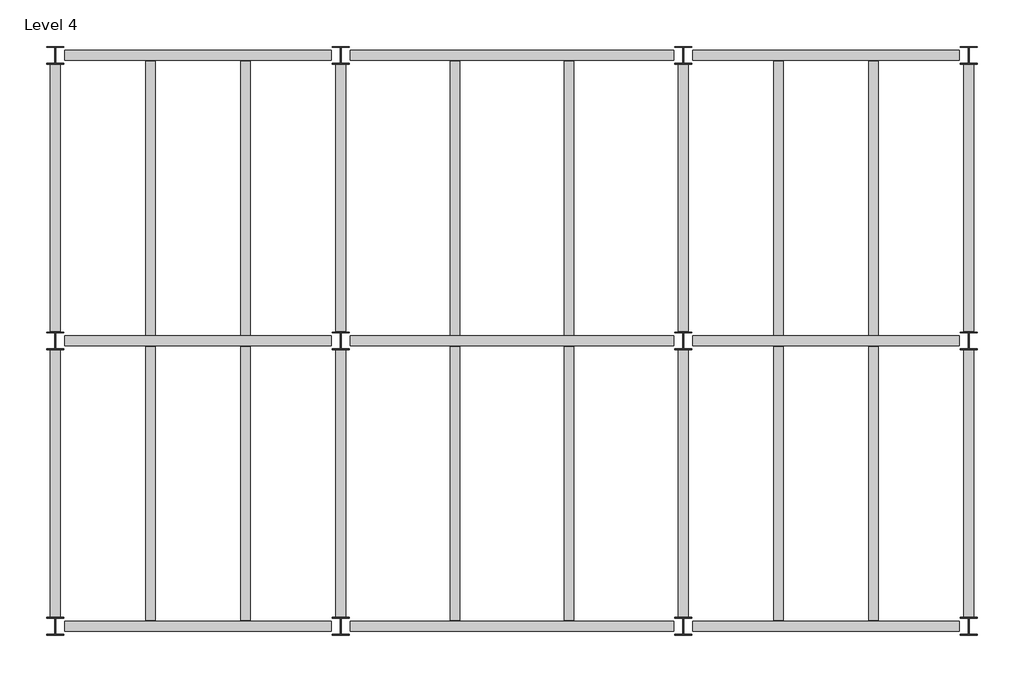
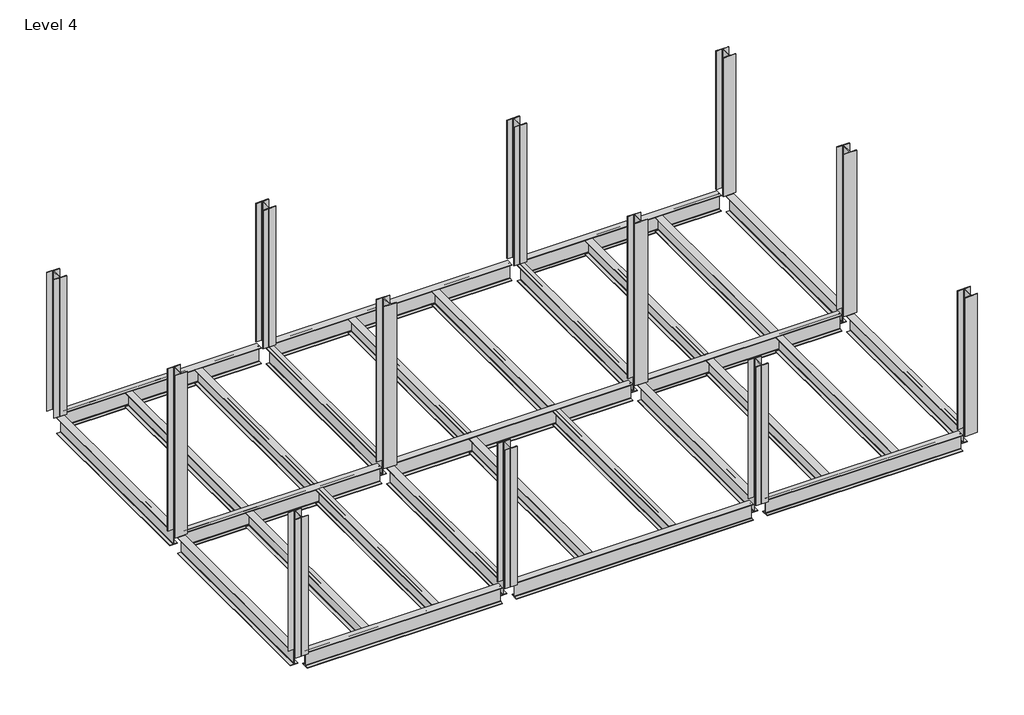
# One storey: 29 beams, 12 columns.
"""IFC4 building model written with IfcOpenShell, lengths in millimetres."""

import ifcopenshell
import ifcopenshell.guid

model = None  # the IFC model being written
_history = None  # IfcOwnerHistory: only IFC2X3 demands one
_inside = {}  # id of a spatial element -> (the spatial element, [elements in it])
_under = {}  # id of a project, library or spatial element -> (it, [spatial elements below it])
_declared = {}  # id of a project -> (the project, [libraries it declares])
_typed = {}  # id of a type object -> (the type object, [elements of that type])
_made_of = {}  # id of a material, layer set ... -> (it, [elements and type objects made of it])


def new_model(schema):
    """Start an empty IFC model of exactly this schema.

    Asked for "IFC4X3", IfcOpenShell would pick the latest addendum, in which some entities
    have other attributes; the version numbers below select the first issue.
    IFC2X3 requires an IfcOwnerHistory on every rooted entity: one is made here for all.
    """
    global model, _history
    if schema == "IFC4X3":
        model = ifcopenshell.file(schema_version=(4, 3, 0, 0))
    else:
        model = ifcopenshell.file(schema=schema)
    _inside.clear()
    _under.clear()
    _declared.clear()
    _typed.clear()
    _made_of.clear()
    _history = None
    if model.schema == "IFC2X3":
        org = make("IfcOrganization", Name="unknown")
        user = make(
            "IfcPersonAndOrganization",
            ThePerson=make("IfcPerson", FamilyName="unknown"),
            TheOrganization=org,
        )
        app = make(
            "IfcApplication",
            ApplicationDeveloper=org,
            Version="unknown",
            ApplicationFullName="unknown",
            ApplicationIdentifier="unknown",
        )
        _history = make(
            "IfcOwnerHistory",
            OwningUser=user,
            OwningApplication=app,
            ChangeAction="ADDED",
            CreationDate=0,
        )
    return model


def make(cls, **values):
    """One entity of the class cls with the attributes given. An attribute that is None is left unset."""
    return model.create_entity(
        cls, **{name: value for name, value in values.items() if value is not None}
    )


def rooted(cls, **values):
    """An entity with a GlobalId (a new one), such as an element, a storey or a relation."""
    return make(cls, GlobalId=ifcopenshell.guid.new(), OwnerHistory=_history, **values)


def si_unit(unit_type, name, prefix=None):
    """IfcSIUnit, for example si_unit("LENGTHUNIT", "METRE", prefix="MILLI")."""
    return make("IfcSIUnit", UnitType=unit_type, Prefix=prefix, Name=name)


def assignment(units):
    """IfcUnitAssignment: the units of a project."""
    return None if units is None else make("IfcUnitAssignment", Units=units)


def point(xyz):
    """IfcCartesianPoint."""
    return None if xyz is None else make("IfcCartesianPoint", Coordinates=xyz)


def direction(xyz):
    """IfcDirection."""
    return None if xyz is None else make("IfcDirection", DirectionRatios=xyz)


def frame(location, z_axis=None, x_axis=None):
    """IfcAxis2Placement3D, a coordinate frame: its origin and axes. An axis left out is left unset."""
    return make(
        "IfcAxis2Placement3D",
        Location=point(location),
        Axis=direction(z_axis),
        RefDirection=direction(x_axis),
    )


def frame_2d(location, x_axis=None):
    """IfcAxis2Placement2D, a coordinate frame in the plane: its origin and x axis."""
    return make(
        "IfcAxis2Placement2D", Location=point(location), RefDirection=direction(x_axis)
    )


def origin():
    """The frame at (0, 0, 0) with its axes left unset."""
    return frame((0.0, 0.0, 0.0))


def place(relative_to, where):
    """IfcLocalPlacement: puts the frame where relative to a parent placement (None: the world)."""
    return make(
        "IfcLocalPlacement", PlacementRelTo=relative_to, RelativePlacement=where
    )


def context(
    kind, dimensions, precision=None, world=None, true_north=None, identifier=None
):
    """IfcGeometricRepresentationContext, for example the 3D "Model" context."""
    return make(
        "IfcGeometricRepresentationContext",
        ContextIdentifier=identifier,
        ContextType=kind,
        CoordinateSpaceDimension=dimensions,
        Precision=precision,
        WorldCoordinateSystem=world,
        TrueNorth=true_north,
    )


def project(units=None, contexts=None):
    """IfcProject with its units and contexts."""
    return rooted(
        "IfcProject",
        Name="project",
        RepresentationContexts=contexts,
        UnitsInContext=assignment(units),
    )


def spatial(cls, under=None, at=None, **own):
    """A site, building, storey or space (cls), placed at a placement, below another one or the project."""
    s = rooted(cls, ObjectPlacement=at, **own)
    if under is not None:
        _under.setdefault(under.id(), (under, []))[1].append(s)
    return s


def polyline(points):
    """IfcPolyline through the points."""
    return make("IfcPolyline", Points=[point(p) for p in points])


def circle_curve(where, radius):
    """IfcCircle in the frame where."""
    return make("IfcCircle", Position=where, Radius=radius)


def trimmed(basis, trim1, trim2, sense, master):
    """IfcTrimmedCurve: the piece of a basis curve between two trims."""
    return make(
        "IfcTrimmedCurve",
        BasisCurve=basis,
        Trim1=trim1,
        Trim2=trim2,
        SenseAgreement=sense,
        MasterRepresentation=master,
    )


def segment(curve, same_sense, transition):
    """IfcCompositeCurveSegment."""
    return make(
        "IfcCompositeCurveSegment",
        Transition=transition,
        SameSense=same_sense,
        ParentCurve=curve,
    )


def composite_curve(segments, self_intersect=None):
    """IfcCompositeCurve: segments joined end to end."""
    return make("IfcCompositeCurve", Segments=segments, SelfIntersect=self_intersect)


def outline(outer, holes=None, kind="AREA"):
    """IfcArbitraryClosedProfileDef: a profile drawn as a closed curve; with holes, ...WithVoids."""
    if holes is None:
        return make("IfcArbitraryClosedProfileDef", ProfileType=kind, OuterCurve=outer)
    return make(
        "IfcArbitraryProfileDefWithVoids",
        ProfileType=kind,
        OuterCurve=outer,
        InnerCurves=holes,
    )


def extrude(swept, where, along, depth):
    """IfcExtrudedAreaSolid: the profile swept, set in the frame where, extruded along a direction by depth."""
    return make(
        "IfcExtrudedAreaSolid",
        SweptArea=swept,
        Position=where,
        ExtrudedDirection=direction(along),
        Depth=depth,
    )


def shape(context_of_items, identifier, shape_type, items):
    """IfcShapeRepresentation: the items that make up one representation, for example the "Body"."""
    return make(
        "IfcShapeRepresentation",
        ContextOfItems=context_of_items,
        RepresentationIdentifier=identifier,
        RepresentationType=shape_type,
        Items=items,
    )


def source(mapping_origin, context_of_items, identifier, shape_type, items):
    """IfcRepresentationMap: a shape defined once, which mapped items show again and again."""
    return make(
        "IfcRepresentationMap",
        MappingOrigin=mapping_origin,
        MappedRepresentation=shape(context_of_items, identifier, shape_type, items),
    )


def transform(
    local_origin,
    x_axis=None,
    y_axis=None,
    z_axis=None,
    scale=None,
    scale2=None,
    scale3=None,
    uniform=True,
):
    """IfcCartesianTransformationOperator3D, or its non-uniform kind. x_axis, y_axis, z_axis: its Axis1, 2, 3."""
    if uniform:
        return make(
            "IfcCartesianTransformationOperator3D",
            Axis1=direction(x_axis),
            Axis2=direction(y_axis),
            LocalOrigin=point(local_origin),
            Scale=scale,
            Axis3=direction(z_axis),
        )
    return make(
        "IfcCartesianTransformationOperator3DnonUniform",
        Axis1=direction(x_axis),
        Axis2=direction(y_axis),
        LocalOrigin=point(local_origin),
        Scale=scale,
        Axis3=direction(z_axis),
        Scale2=scale2,
        Scale3=scale3,
    )


def mapped(mapping_source, mapping_target):
    """IfcMappedItem: shows the shape of a source again, moved by a transform."""
    return make(
        "IfcMappedItem", MappingSource=mapping_source, MappingTarget=mapping_target
    )


def made_of(thing, what):
    """Note that an element or type object is made of a material, layer set ...; save() writes the relation."""
    if what is not None:
        _made_of.setdefault(what.id(), (what, []))[1].append(thing)
    return thing


def element(
    cls,
    number,
    at=None,
    inside=None,
    cuts=None,
    type_object=None,
    material=None,
    context=None,
    identifier="Body",
    shape_type=None,
    held_by="IfcProductDefinitionShape",
    body=None,
    shapes=None,
    **own,
):
    """One element of the class cls, such as IfcWall. Its Tag is "e" and its number.

    at: its placement. inside: the storey or other place that contains it. cuts: it is an
    opening in that element (IfcRelVoidsElement). A single representation is given by context,
    identifier, shape_type and body (its items); several are given by shapes. held_by: the class
    of the entity that holds the representations. save() writes the other relations.
    """
    e = rooted(cls, Tag="e%d" % number, ObjectPlacement=at, **own)
    if body is not None:
        shapes = [shape(context, identifier, shape_type, body)]
    if shapes is not None:
        e.Representation = make(held_by, Representations=shapes)
    if inside is not None:
        _inside.setdefault(inside.id(), (inside, []))[1].append(e)
    if cuts is not None:
        rooted(
            "IfcRelVoidsElement", RelatingBuildingElement=cuts, RelatedOpeningElement=e
        )
    if type_object is not None:
        _typed.setdefault(type_object.id(), (type_object, []))[1].append(e)
    return made_of(e, material)


def aggregate(whole, parts):
    """IfcRelAggregates: a whole, such as a stair, and the parts it consists of."""
    return rooted("IfcRelAggregates", RelatingObject=whole, RelatedObjects=parts)


def save(model, path):
    """Write the relations noted so far, then the file.

    IfcRelAggregates (storeys below a building ...), IfcRelContainedInSpatialStructure (elements
    in a storey), IfcRelDefinesByType, IfcRelAssociatesMaterial and IfcRelDeclares: one each for
    every whole, place, type object, material and project.
    """
    for whole, parts in _under.values():
        aggregate(whole, parts)
    for where, things in _inside.values():
        rooted(
            "IfcRelContainedInSpatialStructure",
            RelatedElements=things,
            RelatingStructure=where,
        )
    for kind, things in _typed.values():
        rooted("IfcRelDefinesByType", RelatedObjects=things, RelatingType=kind)
    for what, things in _made_of.values():
        rooted("IfcRelAssociatesMaterial", RelatedObjects=things, RelatingMaterial=what)
    for by, libraries in _declared.values():
        rooted("IfcRelDeclares", RelatingContext=by, RelatedDefinitions=libraries)
    model.write(path)


def ub_universal_beams_ub356x171x51_26e98692(model_context):
    return source(origin(), model_context, "Body", "SweptSolid", [
        extrude(outline(composite_curve([segment(polyline([(85.75, -166.0), (85.75, -177.5), (-85.75, -177.5), (-85.75, -166.0), (-13.9, -166.0)]), True, "CONTINUOUS"), segment(trimmed(circle_curve(frame_2d((-13.9, -155.8)), 10.2), [point((-13.9, -166.0))], [point((-3.7, -155.8))], True, "CARTESIAN"), True, "CONTINUOUS"), segment(polyline([(-3.7, -155.8), (-3.7, 155.8)]), True, "CONTINUOUS"), segment(trimmed(circle_curve(frame_2d((-13.9, 155.8)), 10.2), [point((-3.7, 155.8))], [point((-13.9, 166.0))], True, "CARTESIAN"), True, "CONTINUOUS"), segment(polyline([(-13.9, 166.0), (-85.75, 166.0), (-85.75, 177.5), (85.75, 177.5), (85.75, 166.0), (13.9, 166.0)]), True, "CONTINUOUS"), segment(trimmed(circle_curve(frame_2d((13.9, 155.8)), 10.2), [point((13.9, 166.0))], [point((3.7, 155.8))], True, "CARTESIAN"), True, "CONTINUOUS"), segment(polyline([(3.7, 155.8), (3.7, -155.8)]), True, "CONTINUOUS"), segment(trimmed(circle_curve(frame_2d((13.9, -155.8)), 10.2), [point((3.7, -155.8))], [point((13.9, -166.0))], True, "CARTESIAN"), True, "CONTINUOUS"), segment(polyline([(13.9, -166.0), (85.75, -166.0)]), True, "CONTINUOUS")], self_intersect=False)), frame((-2398.3, 0.0, 0.0), z_axis=(1.0, 0.0, 0.0), x_axis=(0.0, 1.0, 0.0)), (0.0, 0.0, 1.0), 4796.6),
    ])


def ub_universal_beams_ub406x178x60_425a89a6(model_context):
    return source(origin(), model_context, "Body", "SweptSolid", [
        extrude(outline(composite_curve([segment(polyline([(88.95, -190.4), (88.95, -203.2), (-88.95, -203.2), (-88.95, -190.4), (-14.15, -190.4)]), True, "CONTINUOUS"), segment(trimmed(circle_curve(frame_2d((-14.15, -180.2)), 10.2), [point((-14.15, -190.4))], [point((-3.95, -180.2))], True, "CARTESIAN"), True, "CONTINUOUS"), segment(polyline([(-3.95, -180.2), (-3.95, 180.2)]), True, "CONTINUOUS"), segment(trimmed(circle_curve(frame_2d((-14.15, 180.2)), 10.2), [point((-3.95, 180.2))], [point((-14.15, 190.4))], True, "CARTESIAN"), True, "CONTINUOUS"), segment(polyline([(-14.15, 190.4), (-88.95, 190.4), (-88.95, 203.2), (88.95, 203.2), (88.95, 190.4), (14.15, 190.4)]), True, "CONTINUOUS"), segment(trimmed(circle_curve(frame_2d((14.15, 180.2)), 10.2), [point((14.15, 190.4))], [point((3.95, 180.2))], True, "CARTESIAN"), True, "CONTINUOUS"), segment(polyline([(3.95, 180.2), (3.95, -180.2)]), True, "CONTINUOUS"), segment(trimmed(circle_curve(frame_2d((14.15, -180.2)), 10.2), [point((3.95, -180.2))], [point((14.15, -190.4))], True, "CARTESIAN"), True, "CONTINUOUS"), segment(polyline([(14.15, -190.4), (88.95, -190.4)]), True, "CONTINUOUS")], self_intersect=False)), frame((-2334.6, 0.0, 0.0), z_axis=(1.0, 0.0, 0.0), x_axis=(0.0, 1.0, 0.0)), (0.0, 0.0, 1.0), 4669.2),
    ])


def ub_universal_beams_ub406x178x60_ab0c7e2f(model_context):
    return source(origin(), model_context, "Body", "SweptSolid", [
        extrude(outline(composite_curve([segment(polyline([(88.95, -190.4), (88.95, -203.2), (-88.95, -203.2), (-88.95, -190.4), (-14.15, -190.4)]), True, "CONTINUOUS"), segment(trimmed(circle_curve(frame_2d((-14.15, -180.2)), 10.2), [point((-14.15, -190.4))], [point((-3.95, -180.2))], True, "CARTESIAN"), True, "CONTINUOUS"), segment(polyline([(-3.95, -180.2), (-3.95, 180.2)]), True, "CONTINUOUS"), segment(trimmed(circle_curve(frame_2d((-14.15, 180.2)), 10.2), [point((-3.95, 180.2))], [point((-14.15, 190.4))], True, "CARTESIAN"), True, "CONTINUOUS"), segment(polyline([(-14.15, 190.4), (-88.95, 190.4), (-88.95, 203.2), (88.95, 203.2), (88.95, 190.4), (14.15, 190.4)]), True, "CONTINUOUS"), segment(trimmed(circle_curve(frame_2d((14.15, 180.2)), 10.2), [point((14.15, 190.4))], [point((3.95, 180.2))], True, "CARTESIAN"), True, "CONTINUOUS"), segment(polyline([(3.95, 180.2), (3.95, -180.2)]), True, "CONTINUOUS"), segment(trimmed(circle_curve(frame_2d((14.15, -180.2)), 10.2), [point((3.95, -180.2))], [point((14.15, -190.4))], True, "CARTESIAN"), True, "CONTINUOUS"), segment(polyline([(14.15, -190.4), (88.95, -190.4)]), True, "CONTINUOUS")], self_intersect=False)), frame((-2834.6, 0.0, 0.0), z_axis=(1.0, 0.0, 0.0), x_axis=(0.0, 1.0, 0.0)), (0.0, 0.0, 1.0), 5669.2),
    ])


def ub_universal_beams_ub406x178x60_873acc54(model_context):
    return source(origin(), model_context, "Body", "SweptSolid", [
        extrude(outline(composite_curve([segment(polyline([(88.95, -190.4), (88.95, -203.2), (-88.95, -203.2), (-88.95, -190.4), (-14.15, -190.4)]), True, "CONTINUOUS"), segment(trimmed(circle_curve(frame_2d((-14.15, -180.2)), 10.2), [point((-14.15, -190.4))], [point((-3.95, -180.2))], True, "CARTESIAN"), True, "CONTINUOUS"), segment(polyline([(-3.95, -180.2), (-3.95, 180.2)]), True, "CONTINUOUS"), segment(trimmed(circle_curve(frame_2d((-14.15, 180.2)), 10.2), [point((-3.95, 180.2))], [point((-14.15, 190.4))], True, "CARTESIAN"), True, "CONTINUOUS"), segment(polyline([(-14.15, 190.4), (-88.95, 190.4), (-88.95, 203.2), (88.95, 203.2), (88.95, 190.4), (14.15, 190.4)]), True, "CONTINUOUS"), segment(trimmed(circle_curve(frame_2d((14.15, 180.2)), 10.2), [point((14.15, 190.4))], [point((3.95, 180.2))], True, "CARTESIAN"), True, "CONTINUOUS"), segment(polyline([(3.95, 180.2), (3.95, -180.2)]), True, "CONTINUOUS"), segment(trimmed(circle_curve(frame_2d((14.15, -180.2)), 10.2), [point((3.95, -180.2))], [point((14.15, -190.4))], True, "CARTESIAN"), True, "CONTINUOUS"), segment(polyline([(14.15, -190.4), (88.95, -190.4)]), True, "CONTINUOUS")], self_intersect=False)), frame((-2333.3, 0.0, 0.0), z_axis=(1.0, 0.0, 0.0), x_axis=(0.0, 1.0, 0.0)), (0.0, 0.0, 1.0), 4666.6),
    ])


model = new_model("IFC4")

# Units and contexts
model_context = context("Model", 3, world=origin())
ifc_project = project(units=[si_unit("LENGTHUNIT", "METRE", prefix="MILLI")], contexts=[model_context])

# Site, building, storey
site = spatial("IfcSite", under=ifc_project)
building = spatial("IfcBuilding", under=site)
storey = spatial("IfcBuildingStorey", under=building, Name="Level 4", Elevation=9000.0)

# Beams
placement = place(None, origin())
ub_universal_beams_ub356x171x51_shape = ub_universal_beams_ub356x171x51_26e98692(model_context)
element("IfcBeam", 1, ObjectType="UB-Universal Beams : UB356x171x51", at=placement, inside=storey, context=model_context, shape_type="MappedRepresentation", body=[
    mapped(ub_universal_beams_ub356x171x51_shape, transform((1666.6666667, 2500.0, 8822.5), x_axis=(0.0, 1.0, 0.0), y_axis=(-1.0, 0.0, 0.0), z_axis=(0.0, 0.0, 1.0))),
])
element("IfcBeam", 2, ObjectType="UB-Universal Beams : UB356x171x51", at=placement, inside=storey, context=model_context, shape_type="MappedRepresentation", body=[
    mapped(ub_universal_beams_ub356x171x51_shape, transform((3333.3333333, 2500.0, 8822.5), x_axis=(0.0, 1.0, 0.0), y_axis=(-1.0, 0.0, 0.0), z_axis=(0.0, 0.0, 1.0))),
])
element("IfcBeam", 3, ObjectType="UB-Universal Beams : UB356x171x51", at=placement, inside=storey, context=model_context, shape_type="MappedRepresentation", body=[
    mapped(ub_universal_beams_ub356x171x51_shape, transform((7000.0, 2500.0, 8822.5), x_axis=(0.0, 1.0, 0.0), y_axis=(-1.0, 0.0, 0.0), z_axis=(0.0, 0.0, 1.0))),
])
element("IfcBeam", 4, ObjectType="UB-Universal Beams : UB356x171x51", at=placement, inside=storey, context=model_context, shape_type="MappedRepresentation", body=[
    mapped(ub_universal_beams_ub356x171x51_shape, transform((9000.0, 2500.0, 8822.5), x_axis=(0.0, 1.0, 0.0), y_axis=(-1.0, 0.0, 0.0), z_axis=(0.0, 0.0, 1.0))),
])
element("IfcBeam", 5, ObjectType="UB-Universal Beams : UB356x171x51", at=placement, inside=storey, context=model_context, shape_type="MappedRepresentation", body=[
    mapped(ub_universal_beams_ub356x171x51_shape, transform((12666.6666667, 2500.0, 8822.5), x_axis=(0.0, 1.0, 0.0), y_axis=(-1.0, 0.0, 0.0), z_axis=(0.0, 0.0, 1.0))),
])
element("IfcBeam", 6, ObjectType="UB-Universal Beams : UB356x171x51", at=placement, inside=storey, context=model_context, shape_type="MappedRepresentation", body=[
    mapped(ub_universal_beams_ub356x171x51_shape, transform((14333.3333333, 2500.0, 8822.5), x_axis=(0.0, 1.0, 0.0), y_axis=(-1.0, 0.0, 0.0), z_axis=(0.0, 0.0, 1.0))),
])
element("IfcBeam", 7, ObjectType="UB-Universal Beams : UB356x171x51", at=placement, inside=storey, context=model_context, shape_type="MappedRepresentation", body=[
    mapped(ub_universal_beams_ub356x171x51_shape, transform((1666.6666667, 7500.0, 8822.5), x_axis=(0.0, 1.0, 0.0), y_axis=(-1.0, 0.0, 0.0), z_axis=(0.0, 0.0, 1.0))),
])
element("IfcBeam", 8, ObjectType="UB-Universal Beams : UB356x171x51", at=placement, inside=storey, context=model_context, shape_type="MappedRepresentation", body=[
    mapped(ub_universal_beams_ub356x171x51_shape, transform((3333.3333333, 7500.0, 8822.5), x_axis=(0.0, 1.0, 0.0), y_axis=(-1.0, 0.0, 0.0), z_axis=(0.0, 0.0, 1.0))),
])
element("IfcBeam", 9, ObjectType="UB-Universal Beams : UB356x171x51", at=placement, inside=storey, context=model_context, shape_type="MappedRepresentation", body=[
    mapped(ub_universal_beams_ub356x171x51_shape, transform((7000.0, 7500.0, 8822.5), x_axis=(0.0, 1.0, 0.0), y_axis=(-1.0, 0.0, 0.0), z_axis=(0.0, 0.0, 1.0))),
])
element("IfcBeam", 10, ObjectType="UB-Universal Beams : UB356x171x51", at=placement, inside=storey, context=model_context, shape_type="MappedRepresentation", body=[
    mapped(ub_universal_beams_ub356x171x51_shape, transform((9000.0, 7500.0, 8822.5), x_axis=(0.0, 1.0, 0.0), y_axis=(-1.0, 0.0, 0.0), z_axis=(0.0, 0.0, 1.0))),
])
element("IfcBeam", 11, ObjectType="UB-Universal Beams : UB356x171x51", at=placement, inside=storey, context=model_context, shape_type="MappedRepresentation", body=[
    mapped(ub_universal_beams_ub356x171x51_shape, transform((12666.6666667, 7500.0, 8822.5), x_axis=(0.0, 1.0, 0.0), y_axis=(-1.0, 0.0, 0.0), z_axis=(0.0, 0.0, 1.0))),
])
element("IfcBeam", 12, ObjectType="UB-Universal Beams : UB356x171x51", at=placement, inside=storey, context=model_context, shape_type="MappedRepresentation", body=[
    mapped(ub_universal_beams_ub356x171x51_shape, transform((14333.3333333, 7500.0, 8822.5), x_axis=(0.0, 1.0, 0.0), y_axis=(-1.0, 0.0, 0.0), z_axis=(0.0, 0.0, 1.0))),
])
ub_universal_beams_ub406x178x60_shape = ub_universal_beams_ub406x178x60_425a89a6(model_context)
element("IfcBeam", 13, ObjectType="UB-Universal Beams : UB406x178x60", at=placement, inside=storey, context=model_context, shape_type="MappedRepresentation", body=[
    mapped(ub_universal_beams_ub406x178x60_shape, transform((2500.0, 0.0, 8796.8), x_axis=(1.0, 0.0, 0.0), y_axis=(0.0, 1.0, 0.0), z_axis=(0.0, 0.0, 1.0))),
])
element("IfcBeam", 14, ObjectType="UB-Universal Beams : UB406x178x60", at=placement, inside=storey, context=model_context, shape_type="MappedRepresentation", body=[
    mapped(ub_universal_beams_ub406x178x60_shape, transform((13500.0, 0.0, 8796.8), x_axis=(1.0, 0.0, 0.0), y_axis=(0.0, 1.0, 0.0), z_axis=(0.0, 0.0, 1.0))),
])
element("IfcBeam", 15, ObjectType="UB-Universal Beams : UB406x178x60", at=placement, inside=storey, context=model_context, shape_type="MappedRepresentation", body=[
    mapped(ub_universal_beams_ub406x178x60_shape, transform((2500.0, 5000.0, 8796.8), x_axis=(1.0, 0.0, 0.0), y_axis=(0.0, 1.0, 0.0), z_axis=(0.0, 0.0, 1.0))),
])
element("IfcBeam", 16, ObjectType="UB-Universal Beams : UB406x178x60", at=placement, inside=storey, context=model_context, shape_type="MappedRepresentation", body=[
    mapped(ub_universal_beams_ub406x178x60_shape, transform((13500.0, 5000.0, 8796.8), x_axis=(1.0, 0.0, 0.0), y_axis=(0.0, 1.0, 0.0), z_axis=(0.0, 0.0, 1.0))),
])
element("IfcBeam", 17, ObjectType="UB-Universal Beams : UB406x178x60", at=placement, inside=storey, context=model_context, shape_type="MappedRepresentation", body=[
    mapped(ub_universal_beams_ub406x178x60_shape, transform((2500.0, 10000.0, 8796.8), x_axis=(1.0, 0.0, 0.0), y_axis=(0.0, 1.0, 0.0), z_axis=(0.0, 0.0, 1.0))),
])
element("IfcBeam", 18, ObjectType="UB-Universal Beams : UB406x178x60", at=placement, inside=storey, context=model_context, shape_type="MappedRepresentation", body=[
    mapped(ub_universal_beams_ub406x178x60_shape, transform((13500.0, 10000.0, 8796.8), x_axis=(1.0, 0.0, 0.0), y_axis=(0.0, 1.0, 0.0), z_axis=(0.0, 0.0, 1.0))),
])
ub_universal_beams_ub406x178x60_2_shape = ub_universal_beams_ub406x178x60_ab0c7e2f(model_context)
element("IfcBeam", 19, ObjectType="UB-Universal Beams : UB406x178x60", at=placement, inside=storey, context=model_context, shape_type="MappedRepresentation", body=[
    mapped(ub_universal_beams_ub406x178x60_2_shape, transform((8000.0, 0.0, 8796.8), x_axis=(1.0, 0.0, 0.0), y_axis=(0.0, 1.0, 0.0), z_axis=(0.0, 0.0, 1.0))),
])
element("IfcBeam", 20, ObjectType="UB-Universal Beams : UB406x178x60", at=placement, inside=storey, context=model_context, shape_type="MappedRepresentation", body=[
    mapped(ub_universal_beams_ub406x178x60_2_shape, transform((8000.0, 5000.0, 8796.8), x_axis=(1.0, 0.0, 0.0), y_axis=(0.0, 1.0, 0.0), z_axis=(0.0, 0.0, 1.0))),
])
element("IfcBeam", 21, ObjectType="UB-Universal Beams : UB406x178x60", at=placement, inside=storey, context=model_context, shape_type="MappedRepresentation", body=[
    mapped(ub_universal_beams_ub406x178x60_2_shape, transform((8000.0, 10000.0, 8796.8), x_axis=(1.0, 0.0, 0.0), y_axis=(0.0, 1.0, 0.0), z_axis=(0.0, 0.0, 1.0))),
])
ub_universal_beams_ub406x178x60_3_shape = ub_universal_beams_ub406x178x60_873acc54(model_context)
element("IfcBeam", 22, ObjectType="UB-Universal Beams : UB406x178x60", at=placement, inside=storey, context=model_context, shape_type="MappedRepresentation", body=[
    mapped(ub_universal_beams_ub406x178x60_3_shape, transform((0.0, 2500.0, 8796.8), x_axis=(0.0, 1.0, 0.0), y_axis=(-1.0, 0.0, 0.0), z_axis=(0.0, 0.0, 1.0))),
])
element("IfcBeam", 23, ObjectType="UB-Universal Beams : UB406x178x60", at=placement, inside=storey, context=model_context, shape_type="MappedRepresentation", body=[
    mapped(ub_universal_beams_ub406x178x60_3_shape, transform((0.0, 7500.0, 8796.8), x_axis=(0.0, 1.0, 0.0), y_axis=(-1.0, 0.0, 0.0), z_axis=(0.0, 0.0, 1.0))),
])
element("IfcBeam", 24, ObjectType="UB-Universal Beams : UB406x178x60", at=placement, inside=storey, context=model_context, shape_type="MappedRepresentation", body=[
    mapped(ub_universal_beams_ub406x178x60_3_shape, transform((5000.0, 2500.0, 8796.8), x_axis=(0.0, 1.0, 0.0), y_axis=(-1.0, 0.0, 0.0), z_axis=(0.0, 0.0, 1.0))),
])
element("IfcBeam", 25, ObjectType="UB-Universal Beams : UB406x178x60", at=placement, inside=storey, context=model_context, shape_type="MappedRepresentation", body=[
    mapped(ub_universal_beams_ub406x178x60_3_shape, transform((5000.0, 7500.0, 8796.8), x_axis=(0.0, 1.0, 0.0), y_axis=(-1.0, 0.0, 0.0), z_axis=(0.0, 0.0, 1.0))),
])
element("IfcBeam", 26, ObjectType="UB-Universal Beams : UB406x178x60", at=placement, inside=storey, context=model_context, shape_type="MappedRepresentation", body=[
    mapped(ub_universal_beams_ub406x178x60_3_shape, transform((11000.0, 2500.0, 8796.8), x_axis=(0.0, 1.0, 0.0), y_axis=(-1.0, 0.0, 0.0), z_axis=(0.0, 0.0, 1.0))),
])
element("IfcBeam", 27, ObjectType="UB-Universal Beams : UB406x178x60", at=placement, inside=storey, context=model_context, shape_type="MappedRepresentation", body=[
    mapped(ub_universal_beams_ub406x178x60_3_shape, transform((11000.0, 7500.0, 8796.8), x_axis=(0.0, 1.0, 0.0), y_axis=(-1.0, 0.0, 0.0), z_axis=(0.0, 0.0, 1.0))),
])
element("IfcBeam", 28, ObjectType="UB-Universal Beams : UB406x178x60", at=placement, inside=storey, context=model_context, shape_type="MappedRepresentation", body=[
    mapped(ub_universal_beams_ub406x178x60_3_shape, transform((16000.0, 2500.0, 8796.8), x_axis=(0.0, 1.0, 0.0), y_axis=(-1.0, 0.0, 0.0), z_axis=(0.0, 0.0, 1.0))),
])
element("IfcBeam", 29, ObjectType="UB-Universal Beams : UB406x178x60", at=placement, inside=storey, context=model_context, shape_type="MappedRepresentation", body=[
    mapped(ub_universal_beams_ub406x178x60_3_shape, transform((16000.0, 7500.0, 8796.8), x_axis=(0.0, 1.0, 0.0), y_axis=(-1.0, 0.0, 0.0), z_axis=(0.0, 0.0, 1.0))),
])

# Columns
element("IfcColumn", 30, ObjectType="UC-Universal Columns-Column : UC305x305x97", at=placement, inside=storey, context=model_context, shape_type="SweptSolid", body=[
    extrude(outline(composite_curve([segment(polyline([(152.65, 153.95), (152.65, 138.55), (20.15, 138.55)]), True, "CONTINUOUS"), segment(trimmed(circle_curve(frame_2d((20.15, 123.35)), 15.2), [point((20.15, 138.55))], [point((4.95, 123.35))], True, "CARTESIAN"), True, "CONTINUOUS"), segment(polyline([(4.95, 123.35), (4.95, -123.35)]), True, "CONTINUOUS"), segment(trimmed(circle_curve(frame_2d((20.15, -123.35)), 15.2), [point((4.95, -123.35))], [point((20.15, -138.55))], True, "CARTESIAN"), True, "CONTINUOUS"), segment(polyline([(20.15, -138.55), (152.65, -138.55), (152.65, -153.95), (-152.65, -153.95), (-152.65, -138.55), (-20.15, -138.55)]), True, "CONTINUOUS"), segment(trimmed(circle_curve(frame_2d((-20.15, -123.35)), 15.2), [point((-20.15, -138.55))], [point((-4.95, -123.35))], True, "CARTESIAN"), True, "CONTINUOUS"), segment(polyline([(-4.95, -123.35), (-4.95, 123.35)]), True, "CONTINUOUS"), segment(trimmed(circle_curve(frame_2d((-20.15, 123.35)), 15.2), [point((-4.95, 123.35))], [point((-20.15, 138.55))], True, "CARTESIAN"), True, "CONTINUOUS"), segment(polyline([(-20.15, 138.55), (-152.65, 138.55), (-152.65, 153.95), (152.65, 153.95)]), True, "CONTINUOUS")], self_intersect=False)), frame((0.0, 0.0, 9000.0), z_axis=(0.0, 0.0, 1.0), x_axis=(1.0, 0.0, 0.0)), (0.0, 0.0, 1.0), 3500.0),
])
element("IfcColumn", 31, ObjectType="UC-Universal Columns-Column : UC305x305x97", at=placement, inside=storey, context=model_context, shape_type="SweptSolid", body=[
    extrude(outline(composite_curve([segment(polyline([(5152.65, 153.95), (5152.65, 138.55), (5020.15, 138.55)]), True, "CONTINUOUS"), segment(trimmed(circle_curve(frame_2d((5020.15, 123.35)), 15.2), [point((5020.15, 138.55))], [point((5004.95, 123.35))], True, "CARTESIAN"), True, "CONTINUOUS"), segment(polyline([(5004.95, 123.35), (5004.95, -123.35)]), True, "CONTINUOUS"), segment(trimmed(circle_curve(frame_2d((5020.15, -123.35)), 15.2), [point((5004.95, -123.35))], [point((5020.15, -138.55))], True, "CARTESIAN"), True, "CONTINUOUS"), segment(polyline([(5020.15, -138.55), (5152.65, -138.55), (5152.65, -153.95), (4847.35, -153.95), (4847.35, -138.55), (4979.85, -138.55)]), True, "CONTINUOUS"), segment(trimmed(circle_curve(frame_2d((4979.85, -123.35)), 15.2), [point((4979.85, -138.55))], [point((4995.05, -123.35))], True, "CARTESIAN"), True, "CONTINUOUS"), segment(polyline([(4995.05, -123.35), (4995.05, 123.35)]), True, "CONTINUOUS"), segment(trimmed(circle_curve(frame_2d((4979.85, 123.35)), 15.2), [point((4995.05, 123.35))], [point((4979.85, 138.55))], True, "CARTESIAN"), True, "CONTINUOUS"), segment(polyline([(4979.85, 138.55), (4847.35, 138.55), (4847.35, 153.95), (5152.65, 153.95)]), True, "CONTINUOUS")], self_intersect=False)), frame((0.0, 0.0, 9000.0), z_axis=(0.0, 0.0, 1.0), x_axis=(1.0, 0.0, 0.0)), (0.0, 0.0, 1.0), 3500.0),
])
element("IfcColumn", 32, ObjectType="UC-Universal Columns-Column : UC305x305x97", at=placement, inside=storey, context=model_context, shape_type="SweptSolid", body=[
    extrude(outline(composite_curve([segment(polyline([(11152.65, 153.95), (11152.65, 138.55), (11020.15, 138.55)]), True, "CONTINUOUS"), segment(trimmed(circle_curve(frame_2d((11020.15, 123.35)), 15.2), [point((11020.15, 138.55))], [point((11004.95, 123.35))], True, "CARTESIAN"), True, "CONTINUOUS"), segment(polyline([(11004.95, 123.35), (11004.95, -123.35)]), True, "CONTINUOUS"), segment(trimmed(circle_curve(frame_2d((11020.15, -123.35)), 15.2), [point((11004.95, -123.35))], [point((11020.15, -138.55))], True, "CARTESIAN"), True, "CONTINUOUS"), segment(polyline([(11020.15, -138.55), (11152.65, -138.55), (11152.65, -153.95), (10847.35, -153.95), (10847.35, -138.55), (10979.85, -138.55)]), True, "CONTINUOUS"), segment(trimmed(circle_curve(frame_2d((10979.85, -123.35)), 15.2), [point((10979.85, -138.55))], [point((10995.05, -123.35))], True, "CARTESIAN"), True, "CONTINUOUS"), segment(polyline([(10995.05, -123.35), (10995.05, 123.35)]), True, "CONTINUOUS"), segment(trimmed(circle_curve(frame_2d((10979.85, 123.35)), 15.2), [point((10995.05, 123.35))], [point((10979.85, 138.55))], True, "CARTESIAN"), True, "CONTINUOUS"), segment(polyline([(10979.85, 138.55), (10847.35, 138.55), (10847.35, 153.95), (11152.65, 153.95)]), True, "CONTINUOUS")], self_intersect=False)), frame((0.0, 0.0, 9000.0), z_axis=(0.0, 0.0, 1.0), x_axis=(1.0, 0.0, 0.0)), (0.0, 0.0, 1.0), 3500.0),
])
element("IfcColumn", 33, ObjectType="UC-Universal Columns-Column : UC305x305x97", at=placement, inside=storey, context=model_context, shape_type="SweptSolid", body=[
    extrude(outline(composite_curve([segment(polyline([(16152.65, 153.95), (16152.65, 138.55), (16020.15, 138.55)]), True, "CONTINUOUS"), segment(trimmed(circle_curve(frame_2d((16020.15, 123.35)), 15.2), [point((16020.15, 138.55))], [point((16004.95, 123.35))], True, "CARTESIAN"), True, "CONTINUOUS"), segment(polyline([(16004.95, 123.35), (16004.95, -123.35)]), True, "CONTINUOUS"), segment(trimmed(circle_curve(frame_2d((16020.15, -123.35)), 15.2), [point((16004.95, -123.35))], [point((16020.15, -138.55))], True, "CARTESIAN"), True, "CONTINUOUS"), segment(polyline([(16020.15, -138.55), (16152.65, -138.55), (16152.65, -153.95), (15847.35, -153.95), (15847.35, -138.55), (15979.85, -138.55)]), True, "CONTINUOUS"), segment(trimmed(circle_curve(frame_2d((15979.85, -123.35)), 15.2), [point((15979.85, -138.55))], [point((15995.05, -123.35))], True, "CARTESIAN"), True, "CONTINUOUS"), segment(polyline([(15995.05, -123.35), (15995.05, 123.35)]), True, "CONTINUOUS"), segment(trimmed(circle_curve(frame_2d((15979.85, 123.35)), 15.2), [point((15995.05, 123.35))], [point((15979.85, 138.55))], True, "CARTESIAN"), True, "CONTINUOUS"), segment(polyline([(15979.85, 138.55), (15847.35, 138.55), (15847.35, 153.95), (16152.65, 153.95)]), True, "CONTINUOUS")], self_intersect=False)), frame((0.0, 0.0, 9000.0), z_axis=(0.0, 0.0, 1.0), x_axis=(1.0, 0.0, 0.0)), (0.0, 0.0, 1.0), 3500.0),
])
element("IfcColumn", 34, ObjectType="UC-Universal Columns-Column : UC305x305x97", at=placement, inside=storey, context=model_context, shape_type="SweptSolid", body=[
    extrude(outline(composite_curve([segment(polyline([(152.65, 5153.95), (152.65, 5138.55), (20.15, 5138.55)]), True, "CONTINUOUS"), segment(trimmed(circle_curve(frame_2d((20.15, 5123.35)), 15.2), [point((20.15, 5138.55))], [point((4.95, 5123.35))], True, "CARTESIAN"), True, "CONTINUOUS"), segment(polyline([(4.95, 5123.35), (4.95, 4876.65)]), True, "CONTINUOUS"), segment(trimmed(circle_curve(frame_2d((20.15, 4876.65)), 15.2), [point((4.95, 4876.65))], [point((20.15, 4861.45))], True, "CARTESIAN"), True, "CONTINUOUS"), segment(polyline([(20.15, 4861.45), (152.65, 4861.45), (152.65, 4846.05), (-152.65, 4846.05), (-152.65, 4861.45), (-20.15, 4861.45)]), True, "CONTINUOUS"), segment(trimmed(circle_curve(frame_2d((-20.15, 4876.65)), 15.2), [point((-20.15, 4861.45))], [point((-4.95, 4876.65))], True, "CARTESIAN"), True, "CONTINUOUS"), segment(polyline([(-4.95, 4876.65), (-4.95, 5123.35)]), True, "CONTINUOUS"), segment(trimmed(circle_curve(frame_2d((-20.15, 5123.35)), 15.2), [point((-4.95, 5123.35))], [point((-20.15, 5138.55))], True, "CARTESIAN"), True, "CONTINUOUS"), segment(polyline([(-20.15, 5138.55), (-152.65, 5138.55), (-152.65, 5153.95), (152.65, 5153.95)]), True, "CONTINUOUS")], self_intersect=False)), frame((0.0, 0.0, 9000.0), z_axis=(0.0, 0.0, 1.0), x_axis=(1.0, 0.0, 0.0)), (0.0, 0.0, 1.0), 4100.0),
])
element("IfcColumn", 35, ObjectType="UC-Universal Columns-Column : UC305x305x97", at=placement, inside=storey, context=model_context, shape_type="SweptSolid", body=[
    extrude(outline(composite_curve([segment(polyline([(5152.65, 5153.95), (5152.65, 5138.55), (5020.15, 5138.55)]), True, "CONTINUOUS"), segment(trimmed(circle_curve(frame_2d((5020.15, 5123.35)), 15.2), [point((5020.15, 5138.55))], [point((5004.95, 5123.35))], True, "CARTESIAN"), True, "CONTINUOUS"), segment(polyline([(5004.95, 5123.35), (5004.95, 4876.65)]), True, "CONTINUOUS"), segment(trimmed(circle_curve(frame_2d((5020.15, 4876.65)), 15.2), [point((5004.95, 4876.65))], [point((5020.15, 4861.45))], True, "CARTESIAN"), True, "CONTINUOUS"), segment(polyline([(5020.15, 4861.45), (5152.65, 4861.45), (5152.65, 4846.05), (4847.35, 4846.05), (4847.35, 4861.45), (4979.85, 4861.45)]), True, "CONTINUOUS"), segment(trimmed(circle_curve(frame_2d((4979.85, 4876.65)), 15.2), [point((4979.85, 4861.45))], [point((4995.05, 4876.65))], True, "CARTESIAN"), True, "CONTINUOUS"), segment(polyline([(4995.05, 4876.65), (4995.05, 5123.35)]), True, "CONTINUOUS"), segment(trimmed(circle_curve(frame_2d((4979.85, 5123.35)), 15.2), [point((4995.05, 5123.35))], [point((4979.85, 5138.55))], True, "CARTESIAN"), True, "CONTINUOUS"), segment(polyline([(4979.85, 5138.55), (4847.35, 5138.55), (4847.35, 5153.95), (5152.65, 5153.95)]), True, "CONTINUOUS")], self_intersect=False)), frame((0.0, 0.0, 9000.0), z_axis=(0.0, 0.0, 1.0), x_axis=(1.0, 0.0, 0.0)), (0.0, 0.0, 1.0), 4100.0),
])
element("IfcColumn", 36, ObjectType="UC-Universal Columns-Column : UC305x305x97", at=placement, inside=storey, context=model_context, shape_type="SweptSolid", body=[
    extrude(outline(composite_curve([segment(polyline([(11152.65, 5153.95), (11152.65, 5138.55), (11020.15, 5138.55)]), True, "CONTINUOUS"), segment(trimmed(circle_curve(frame_2d((11020.15, 5123.35)), 15.2), [point((11020.15, 5138.55))], [point((11004.95, 5123.35))], True, "CARTESIAN"), True, "CONTINUOUS"), segment(polyline([(11004.95, 5123.35), (11004.95, 4876.65)]), True, "CONTINUOUS"), segment(trimmed(circle_curve(frame_2d((11020.15, 4876.65)), 15.2), [point((11004.95, 4876.65))], [point((11020.15, 4861.45))], True, "CARTESIAN"), True, "CONTINUOUS"), segment(polyline([(11020.15, 4861.45), (11152.65, 4861.45), (11152.65, 4846.05), (10847.35, 4846.05), (10847.35, 4861.45), (10979.85, 4861.45)]), True, "CONTINUOUS"), segment(trimmed(circle_curve(frame_2d((10979.85, 4876.65)), 15.2), [point((10979.85, 4861.45))], [point((10995.05, 4876.65))], True, "CARTESIAN"), True, "CONTINUOUS"), segment(polyline([(10995.05, 4876.65), (10995.05, 5123.35)]), True, "CONTINUOUS"), segment(trimmed(circle_curve(frame_2d((10979.85, 5123.35)), 15.2), [point((10995.05, 5123.35))], [point((10979.85, 5138.55))], True, "CARTESIAN"), True, "CONTINUOUS"), segment(polyline([(10979.85, 5138.55), (10847.35, 5138.55), (10847.35, 5153.95), (11152.65, 5153.95)]), True, "CONTINUOUS")], self_intersect=False)), frame((0.0, 0.0, 9000.0), z_axis=(0.0, 0.0, 1.0), x_axis=(1.0, 0.0, 0.0)), (0.0, 0.0, 1.0), 4100.0),
])
element("IfcColumn", 37, ObjectType="UC-Universal Columns-Column : UC305x305x97", at=placement, inside=storey, context=model_context, shape_type="SweptSolid", body=[
    extrude(outline(composite_curve([segment(polyline([(16152.65, 5153.95), (16152.65, 5138.55), (16020.15, 5138.55)]), True, "CONTINUOUS"), segment(trimmed(circle_curve(frame_2d((16020.15, 5123.35)), 15.2), [point((16020.15, 5138.55))], [point((16004.95, 5123.35))], True, "CARTESIAN"), True, "CONTINUOUS"), segment(polyline([(16004.95, 5123.35), (16004.95, 4876.65)]), True, "CONTINUOUS"), segment(trimmed(circle_curve(frame_2d((16020.15, 4876.65)), 15.2), [point((16004.95, 4876.65))], [point((16020.15, 4861.45))], True, "CARTESIAN"), True, "CONTINUOUS"), segment(polyline([(16020.15, 4861.45), (16152.65, 4861.45), (16152.65, 4846.05), (15847.35, 4846.05), (15847.35, 4861.45), (15979.85, 4861.45)]), True, "CONTINUOUS"), segment(trimmed(circle_curve(frame_2d((15979.85, 4876.65)), 15.2), [point((15979.85, 4861.45))], [point((15995.05, 4876.65))], True, "CARTESIAN"), True, "CONTINUOUS"), segment(polyline([(15995.05, 4876.65), (15995.05, 5123.35)]), True, "CONTINUOUS"), segment(trimmed(circle_curve(frame_2d((15979.85, 5123.35)), 15.2), [point((15995.05, 5123.35))], [point((15979.85, 5138.55))], True, "CARTESIAN"), True, "CONTINUOUS"), segment(polyline([(15979.85, 5138.55), (15847.35, 5138.55), (15847.35, 5153.95), (16152.65, 5153.95)]), True, "CONTINUOUS")], self_intersect=False)), frame((0.0, 0.0, 9000.0), z_axis=(0.0, 0.0, 1.0), x_axis=(1.0, 0.0, 0.0)), (0.0, 0.0, 1.0), 4100.0),
])
element("IfcColumn", 38, ObjectType="UC-Universal Columns-Column : UC305x305x97", at=placement, inside=storey, context=model_context, shape_type="SweptSolid", body=[
    extrude(outline(composite_curve([segment(polyline([(152.65, 10153.95), (152.65, 10138.55), (20.15, 10138.55)]), True, "CONTINUOUS"), segment(trimmed(circle_curve(frame_2d((20.15, 10123.35)), 15.2), [point((20.15, 10138.55))], [point((4.95, 10123.35))], True, "CARTESIAN"), True, "CONTINUOUS"), segment(polyline([(4.95, 10123.35), (4.95, 9876.65)]), True, "CONTINUOUS"), segment(trimmed(circle_curve(frame_2d((20.15, 9876.65)), 15.2), [point((4.95, 9876.65))], [point((20.15, 9861.45))], True, "CARTESIAN"), True, "CONTINUOUS"), segment(polyline([(20.15, 9861.45), (152.65, 9861.45), (152.65, 9846.05), (-152.65, 9846.05), (-152.65, 9861.45), (-20.15, 9861.45)]), True, "CONTINUOUS"), segment(trimmed(circle_curve(frame_2d((-20.15, 9876.65)), 15.2), [point((-20.15, 9861.45))], [point((-4.95, 9876.65))], True, "CARTESIAN"), True, "CONTINUOUS"), segment(polyline([(-4.95, 9876.65), (-4.95, 10123.35)]), True, "CONTINUOUS"), segment(trimmed(circle_curve(frame_2d((-20.15, 10123.35)), 15.2), [point((-4.95, 10123.35))], [point((-20.15, 10138.55))], True, "CARTESIAN"), True, "CONTINUOUS"), segment(polyline([(-20.15, 10138.55), (-152.65, 10138.55), (-152.65, 10153.95), (152.65, 10153.95)]), True, "CONTINUOUS")], self_intersect=False)), frame((0.0, 0.0, 9000.0), z_axis=(0.0, 0.0, 1.0), x_axis=(1.0, 0.0, 0.0)), (0.0, 0.0, 1.0), 3500.0),
])
element("IfcColumn", 39, ObjectType="UC-Universal Columns-Column : UC305x305x97", at=placement, inside=storey, context=model_context, shape_type="SweptSolid", body=[
    extrude(outline(composite_curve([segment(polyline([(5152.65, 10153.95), (5152.65, 10138.55), (5020.15, 10138.55)]), True, "CONTINUOUS"), segment(trimmed(circle_curve(frame_2d((5020.15, 10123.35)), 15.2), [point((5020.15, 10138.55))], [point((5004.95, 10123.35))], True, "CARTESIAN"), True, "CONTINUOUS"), segment(polyline([(5004.95, 10123.35), (5004.95, 9876.65)]), True, "CONTINUOUS"), segment(trimmed(circle_curve(frame_2d((5020.15, 9876.65)), 15.2), [point((5004.95, 9876.65))], [point((5020.15, 9861.45))], True, "CARTESIAN"), True, "CONTINUOUS"), segment(polyline([(5020.15, 9861.45), (5152.65, 9861.45), (5152.65, 9846.05), (4847.35, 9846.05), (4847.35, 9861.45), (4979.85, 9861.45)]), True, "CONTINUOUS"), segment(trimmed(circle_curve(frame_2d((4979.85, 9876.65)), 15.2), [point((4979.85, 9861.45))], [point((4995.05, 9876.65))], True, "CARTESIAN"), True, "CONTINUOUS"), segment(polyline([(4995.05, 9876.65), (4995.05, 10123.35)]), True, "CONTINUOUS"), segment(trimmed(circle_curve(frame_2d((4979.85, 10123.35)), 15.2), [point((4995.05, 10123.35))], [point((4979.85, 10138.55))], True, "CARTESIAN"), True, "CONTINUOUS"), segment(polyline([(4979.85, 10138.55), (4847.35, 10138.55), (4847.35, 10153.95), (5152.65, 10153.95)]), True, "CONTINUOUS")], self_intersect=False)), frame((0.0, 0.0, 9000.0), z_axis=(0.0, 0.0, 1.0), x_axis=(1.0, 0.0, 0.0)), (0.0, 0.0, 1.0), 3500.0),
])
element("IfcColumn", 40, ObjectType="UC-Universal Columns-Column : UC305x305x97", at=placement, inside=storey, context=model_context, shape_type="SweptSolid", body=[
    extrude(outline(composite_curve([segment(polyline([(11152.65, 10153.95), (11152.65, 10138.55), (11020.15, 10138.55)]), True, "CONTINUOUS"), segment(trimmed(circle_curve(frame_2d((11020.15, 10123.35)), 15.2), [point((11020.15, 10138.55))], [point((11004.95, 10123.35))], True, "CARTESIAN"), True, "CONTINUOUS"), segment(polyline([(11004.95, 10123.35), (11004.95, 9876.65)]), True, "CONTINUOUS"), segment(trimmed(circle_curve(frame_2d((11020.15, 9876.65)), 15.2), [point((11004.95, 9876.65))], [point((11020.15, 9861.45))], True, "CARTESIAN"), True, "CONTINUOUS"), segment(polyline([(11020.15, 9861.45), (11152.65, 9861.45), (11152.65, 9846.05), (10847.35, 9846.05), (10847.35, 9861.45), (10979.85, 9861.45)]), True, "CONTINUOUS"), segment(trimmed(circle_curve(frame_2d((10979.85, 9876.65)), 15.2), [point((10979.85, 9861.45))], [point((10995.05, 9876.65))], True, "CARTESIAN"), True, "CONTINUOUS"), segment(polyline([(10995.05, 9876.65), (10995.05, 10123.35)]), True, "CONTINUOUS"), segment(trimmed(circle_curve(frame_2d((10979.85, 10123.35)), 15.2), [point((10995.05, 10123.35))], [point((10979.85, 10138.55))], True, "CARTESIAN"), True, "CONTINUOUS"), segment(polyline([(10979.85, 10138.55), (10847.35, 10138.55), (10847.35, 10153.95), (11152.65, 10153.95)]), True, "CONTINUOUS")], self_intersect=False)), frame((0.0, 0.0, 9000.0), z_axis=(0.0, 0.0, 1.0), x_axis=(1.0, 0.0, 0.0)), (0.0, 0.0, 1.0), 3500.0),
])
element("IfcColumn", 41, ObjectType="UC-Universal Columns-Column : UC305x305x97", at=placement, inside=storey, context=model_context, shape_type="SweptSolid", body=[
    extrude(outline(composite_curve([segment(polyline([(16152.65, 10153.95), (16152.65, 10138.55), (16020.15, 10138.55)]), True, "CONTINUOUS"), segment(trimmed(circle_curve(frame_2d((16020.15, 10123.35)), 15.2), [point((16020.15, 10138.55))], [point((16004.95, 10123.35))], True, "CARTESIAN"), True, "CONTINUOUS"), segment(polyline([(16004.95, 10123.35), (16004.95, 9876.65)]), True, "CONTINUOUS"), segment(trimmed(circle_curve(frame_2d((16020.15, 9876.65)), 15.2), [point((16004.95, 9876.65))], [point((16020.15, 9861.45))], True, "CARTESIAN"), True, "CONTINUOUS"), segment(polyline([(16020.15, 9861.45), (16152.65, 9861.45), (16152.65, 9846.05), (15847.35, 9846.05), (15847.35, 9861.45), (15979.85, 9861.45)]), True, "CONTINUOUS"), segment(trimmed(circle_curve(frame_2d((15979.85, 9876.65)), 15.2), [point((15979.85, 9861.45))], [point((15995.05, 9876.65))], True, "CARTESIAN"), True, "CONTINUOUS"), segment(polyline([(15995.05, 9876.65), (15995.05, 10123.35)]), True, "CONTINUOUS"), segment(trimmed(circle_curve(frame_2d((15979.85, 10123.35)), 15.2), [point((15995.05, 10123.35))], [point((15979.85, 10138.55))], True, "CARTESIAN"), True, "CONTINUOUS"), segment(polyline([(15979.85, 10138.55), (15847.35, 10138.55), (15847.35, 10153.95), (16152.65, 10153.95)]), True, "CONTINUOUS")], self_intersect=False)), frame((0.0, 0.0, 9000.0), z_axis=(0.0, 0.0, 1.0), x_axis=(1.0, 0.0, 0.0)), (0.0, 0.0, 1.0), 3500.0),
])

save(model, "model.ifc")

# Revit data of these elements
# Type "UB-Universal Beams : UB356x171x51"
#   Section Name Key = "UB356X171X51"
#   Width = 17.15 cm
#   Web Thickness = 0.74 cm
#   Web Fillet = 1.02 cm
#   Warping Constant = 286000.0 cm⁶
#   Torsional Moment of Inertia = 23.80 cm⁴
#   Section Area = 64.9 cm²
#   Plastic Modulus weak axis = 174.0 cm³
#   Plastic Modulus strong axis = 896.0 cm³
#   Nominal Weight = 50.9998 kgf/m
#   Moment of Inertia weak axis = 968.00 cm⁴
#   Moment of Inertia strong axis = 14136.00 cm⁴
#   Height = 35.5 cm
#   Flange Thickness = 1.15 cm
#   Elastic Modulus weak axis = 113.0 cm³
#   Elastic Modulus strong axis = 796.0 cm³
#   Centroid Vertical = 17.75 cm
#   Centroid Horizontal = 8.575 cm
#   Bolt Spacing = 9.0 cm
#   Length [instance default] = 1500 mm
#   Structural Material [instance default] = Metal - Steel 43-275
#   Type Comments = ""
#   Assembly Code = ""
# Type "UB-Universal Beams : UB406x178x60"
#   Section Name Key = "UB406X178X60"
#   Width = 17.79 cm
#   Web Thickness = 0.79 cm
#   Web Fillet = 1.02 cm
#   Warping Constant = 466000.0 cm⁶
#   Torsional Moment of Inertia = 33.30 cm⁴
#   Section Area = 76.5 cm²
#   Plastic Modulus weak axis = 209.0 cm³
#   Plastic Modulus strong axis = 1200.0 cm³
#   Nominal Weight = 60.0998 kgf/m
#   Moment of Inertia weak axis = 1203.00 cm⁴
#   Moment of Inertia strong axis = 21596.00 cm⁴
#   Height = 40.64 cm
#   Flange Thickness = 1.28 cm
#   Elastic Modulus weak axis = 135.0 cm³
#   Elastic Modulus strong axis = 1063.0 cm³
#   Centroid Vertical = 20.32 cm
#   Centroid Horizontal = 8.895 cm
#   Bolt Spacing = 9.0 cm
#   Length [instance default] = 1500 mm
#   Structural Material [instance default] = Metal - Steel 43-275
#   Type Comments = ""
#   Assembly Code = ""
# Type "UC-Universal Columns-Column : UC305x305x97"
#   Section Name Key = "UC305x305x97"
#   Width = 30.53 cm
#   Web Thickness = 0.99 cm
#   Web Fillet = 1.52 cm
#   Warping Constant = 1560000.0 cm⁶
#   Torsional Moment of Inertia = 91.20 cm⁴
#   Section Area = 123.0 cm²
#   Plastic Modulus weak axis = 726.0 cm³
#   Plastic Modulus strong axis = 1592.0 cm³
#   Nominal Weight = 96.8996 kgf/m
#   Moment of Inertia weak axis = 7308.00 cm⁴
#   Moment of Inertia strong axis = 22249.00 cm⁴
#   Height = 30.79 cm
#   Flange Thickness = 1.54 cm
#   Elastic Modulus weak axis = 479.0 cm³
#   Elastic Modulus strong axis = 1445.0 cm³
#   Centroid Vertical = 15.395 cm
#   Centroid Horizontal = 15.265 cm
#   Bolt Spacing = 14.0 cm
#   Structural Material [instance default] = Metal - Steel 43-275
#   Type Comments = ""
#   Assembly Code = ""
# Elements 1, 2, 3, 4, 5, 6, 7, 8, 9, 10, 11, 12 (IfcBeam, "UB-Universal Beams : UB356x171x51")
#   Structural Material = Metal - Steel 43-275
#   Phase Created = New Construction
#   Materials on its faces: "Metal - Steel 43-275"
# Elements 13, 14, 15, 16, 17, 18, 19, 20, 21, 22, 23, 24, 25, 26, 27, 28, 29 (IfcBeam, "UB-Universal Beams : UB406x178x60")
#   Structural Material = Metal - Steel 43-275
#   Phase Created = New Construction
#   Materials on its faces: "Metal - Steel 43-275"
# Elements 30, 31, 32, 33, 34, 35, 36, 37, 38, 39, 40, 41 (IfcColumn, "UC-Universal Columns-Column : UC305x305x97")
#   Structural Material = Metal - Steel 43-275
#   Phase Created = New Construction
#   Materials on its faces: "Metal - Steel 43-275"
# Materials
#   "Metal - Steel 43-275": class "Metal", colour RGB 247 247 247, transparency 0, Cost = 0
